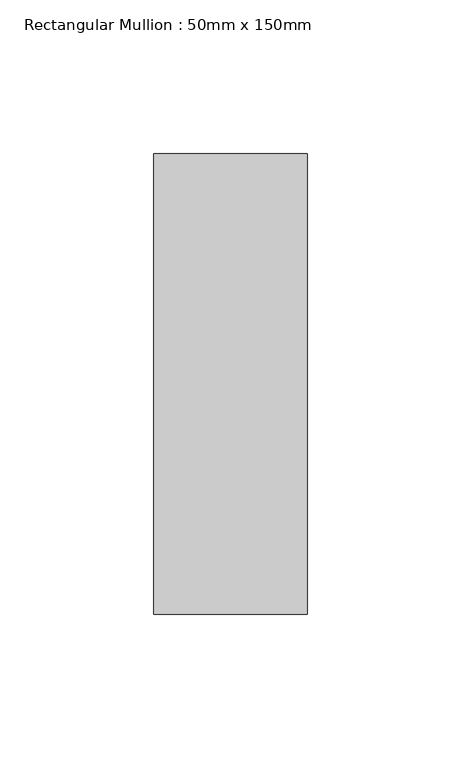
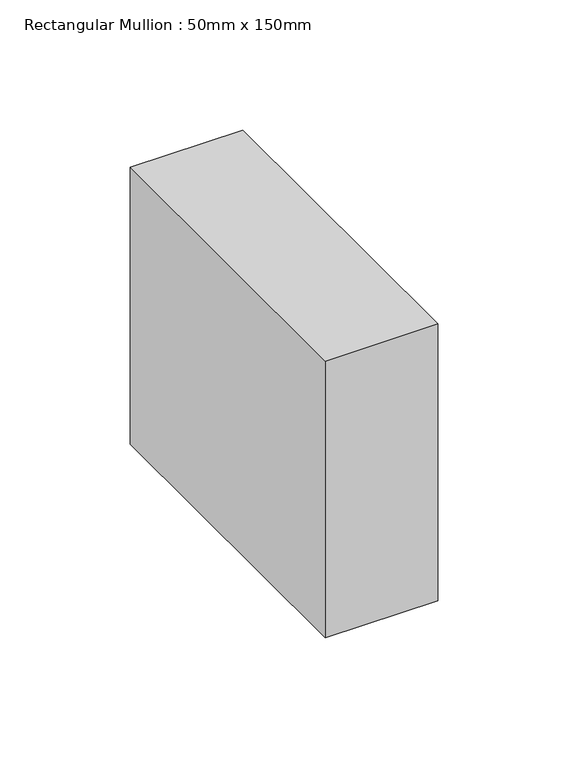
"""IFC4 building model written with IfcOpenShell, lengths in millimetres: member geometry, Rectangular Mullion : 50mm x 150mm."""

from ifc_helpers import new_model, si_unit, frame, origin, place, context, project, spatial, polyline, outline, extrude, source, transform, mapped, element, save


def rectangular_mullion_50mm_x_150mm_da5f7ae8(model_context):
    return source(origin(), model_context, "Body", "SweptSolid", [
        extrude(outline(polyline([(0.0, 75.0), (0.0, -75.0), (-50.0, -75.0), (-50.0, 75.0), (0.0, 75.0)])), frame((0.0, 0.0, -130.0), z_axis=(0.0, 0.0, 1.0), x_axis=(1.0, 0.0, 0.0)), (0.0, 0.0, 1.0), 130.0),
    ])


if __name__ == "__main__":
    model = new_model("IFC4")
    model_context = context("Model", 3, world=origin())
    ifc_project = project(units=[si_unit("LENGTHUNIT", "METRE", prefix="MILLI")], contexts=[model_context])
    site = spatial("IfcSite", under=ifc_project)
    building = spatial("IfcBuilding", under=site)
    placement = place(None, origin())
    rectangular_mullion_50mm_x_150mm_shape = rectangular_mullion_50mm_x_150mm_da5f7ae8(model_context)
    element("IfcMember", 1, ObjectType="Rectangular Mullion : 50mm x 150mm", at=placement, inside=building, context=model_context, shape_type="MappedRepresentation", body=[
        mapped(rectangular_mullion_50mm_x_150mm_shape, transform((0.0, 0.0, 0.0), x_axis=(1.0, 0.0, 0.0), y_axis=(0.0, 1.0, 0.0), z_axis=(0.0, 0.0, 1.0))),
    ])
    save(model, "model.ifc")

# Revit data of these elements
# Type "Rectangular Mullion : 50mm x 150mm"
#   built-in parameter 1007304 = 0.492126 (stored number, unit not read)
#   built-in parameter 1007301 = 0.082021 (stored number, unit not read)
#   built-in parameter 1007300 = 0.082021 (stored number, unit not read)
# Element 1 (IfcMember, "Rectangular Mullion : 50mm x 150mm")
#   Materials on its faces: "Aluminum"
# Materials
#   "Aluminum": class "Metal", colour RGB 244 244 244, transparency 0, Description = "Aluminum 6061", Cost = 0
